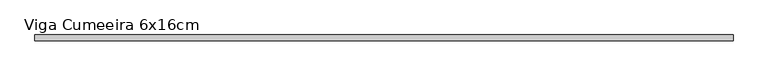
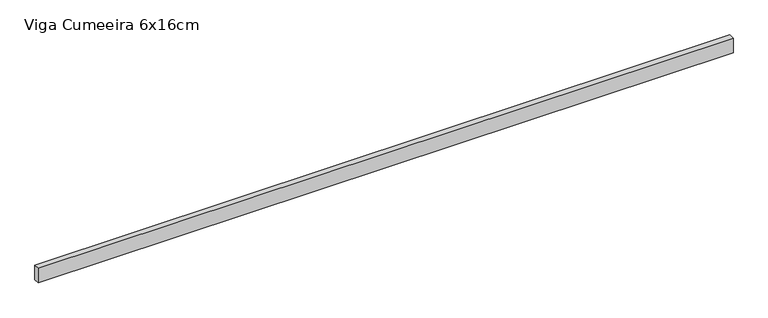
"""IFC4 building model written with IfcOpenShell, lengths in millimetres: beam geometry, Madeira de lei : Viga Cumeeira 6x16cm."""

from ifc_helpers import new_model, si_unit, frame, origin, place, context, project, spatial, polyline, outline, extrude, source, transform, mapped, element, save


def viga_cumeeira_6x16cm_d80f05ee(model_context):
    return source(origin(), model_context, "Body", "SweptSolid", [
        extrude(outline(polyline([(3626.5, 30.0), (3626.5, -30.0), (-3626.5, -30.0), (-3626.5, 30.0), (3626.5, 30.0)])), frame((0.0, 0.0, -80.0), z_axis=(0.0, 0.0, 1.0), x_axis=(1.0, 0.0, 0.0)), (0.0, 0.0, 1.0), 160.0),
    ])


if __name__ == "__main__":
    model = new_model("IFC4")
    model_context = context("Model", 3, world=origin())
    ifc_project = project(units=[si_unit("LENGTHUNIT", "METRE", prefix="MILLI")], contexts=[model_context])
    site = spatial("IfcSite", under=ifc_project)
    building = spatial("IfcBuilding", under=site)
    placement = place(None, origin())
    viga_cumeeira_6x16cm_shape = viga_cumeeira_6x16cm_d80f05ee(model_context)
    element("IfcBeam", 1, ObjectType="Madeira de lei : Viga Cumeeira 6x16cm", at=placement, inside=building, context=model_context, shape_type="MappedRepresentation", body=[
        mapped(viga_cumeeira_6x16cm_shape, transform((0.0, 0.0, 0.0), x_axis=(1.0, 0.0, 0.0), y_axis=(0.0, 1.0, 0.0), z_axis=(0.0, 0.0, 1.0))),
    ])
    save(model, "model.ifc")

# Revit data of these elements
# Type "Madeira de lei : Viga Cumeeira 6x16cm"
#   A = 0.02 m²
#   Length [instance default] = 1.524 m
#   b = 0.06 m
#   d = 0.16 m
#   Structural Material [instance default] = none
#   Assembly Code = ""
# Element 1 (IfcBeam, "Madeira de lei : Viga Cumeeira 6x16cm")
#   Structural Material = .MADEIRAMENTO
#   Materials on its faces: ".MADEIRAMENTO"
# Materials
#   ".MADEIRAMENTO": class ".CC_MADEIRAS", colour RGB 212 179 113, transparency 0, Cost = 0
